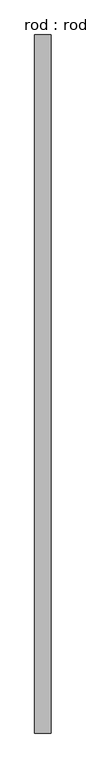
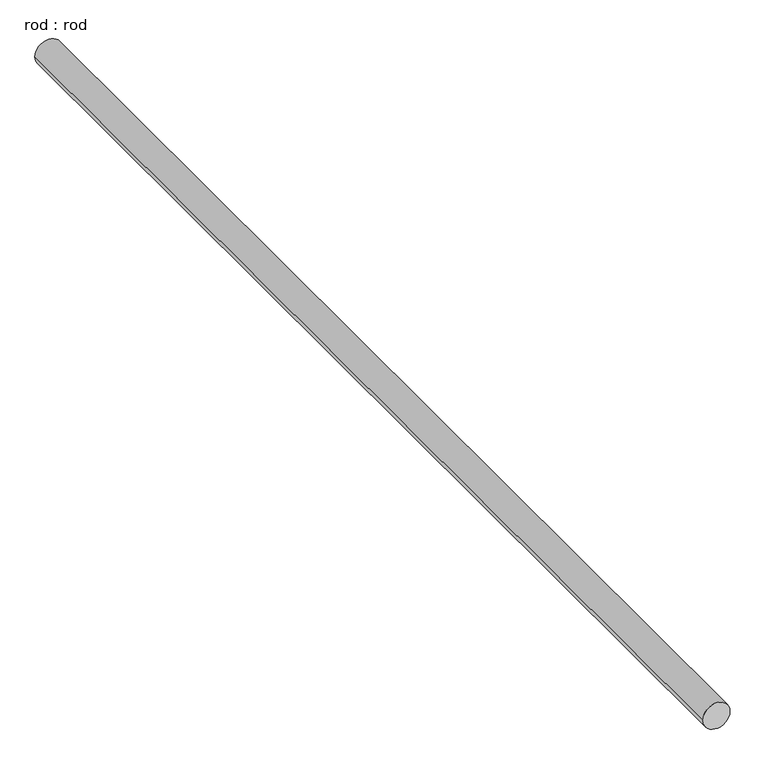
"""IFC4 building model written with IfcOpenShell, lengths in millimetres: proxy geometry, rod : rod."""

from ifc_helpers import new_model, si_unit, point, frame, frame_2d, origin, place, context, project, spatial, circle_curve, trimmed, segment, composite_curve, outline, extrude, source, transform, mapped, element, save


def rod_rod_06da573d(model_context):
    return source(origin(), model_context, "Body", "SweptSolid", [
        extrude(outline(composite_curve([segment(trimmed(circle_curve(frame_2d((0.0108462, 0.0)), 200.0), [point((0.0108462, 200.0))], [point((0.0108462, -200.0))], False, "CARTESIAN"), True, "CONTINUOUS"), segment(trimmed(circle_curve(frame_2d((0.0108462, 0.0)), 200.0), [point((0.0108462, -200.0))], [point((0.0108462, 200.0))], False, "CARTESIAN"), True, "CONTINUOUS")], self_intersect=False)), frame((0.0, -4416.0735334, 0.0), z_axis=(0.0, 1.0, 0.0), x_axis=(0.0, 0.0, 1.0)), (0.0, 0.0, 1.0), 17017.6042975),
    ])


if __name__ == "__main__":
    model = new_model("IFC4")
    model_context = context("Model", 3, world=origin())
    ifc_project = project(units=[si_unit("LENGTHUNIT", "METRE", prefix="MILLI")], contexts=[model_context])
    site = spatial("IfcSite", under=ifc_project)
    building = spatial("IfcBuilding", under=site)
    placement = place(None, origin())
    rod_rod_shape = rod_rod_06da573d(model_context)
    element("IfcBuildingElementProxy", 1, Name="rod : rod", ObjectType="rod : rod", at=placement, inside=building, context=model_context, shape_type="MappedRepresentation", body=[
        mapped(rod_rod_shape, transform((0.0, 0.0, 0.0), x_axis=(1.0, 0.0, 0.0), y_axis=(0.0, 1.0, 0.0), z_axis=(0.0, 0.0, 1.0))),
    ])
    save(model, "model.ifc")

# Revit data of these elements
# Type "rod : rod"
#   Default Elevation = 0
